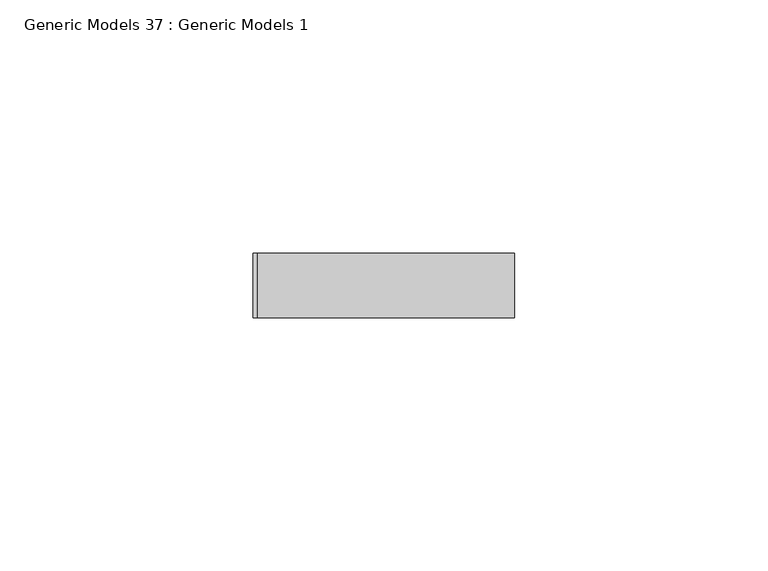
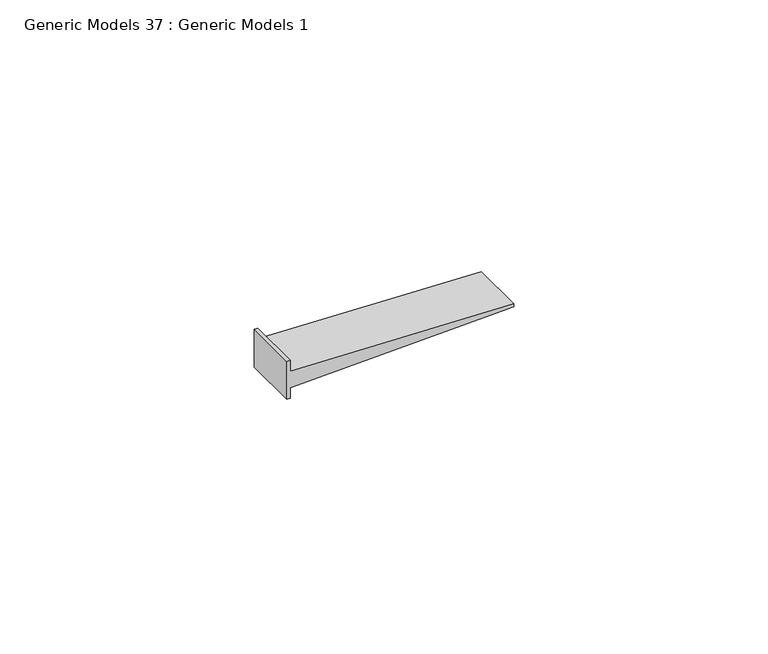
"""IFC4 building model written with IfcOpenShell, lengths in millimetres: proxy geometry, Generic Models 37 : Generic Models 1."""

import ifcopenshell
import ifcopenshell.guid

model = None  # the IFC model being written
_history = None  # IfcOwnerHistory: only IFC2X3 demands one
_inside = {}  # id of a spatial element -> (the spatial element, [elements in it])
_under = {}  # id of a project, library or spatial element -> (it, [spatial elements below it])
_declared = {}  # id of a project -> (the project, [libraries it declares])
_typed = {}  # id of a type object -> (the type object, [elements of that type])
_made_of = {}  # id of a material, layer set ... -> (it, [elements and type objects made of it])


def new_model(schema):
    """Start an empty IFC model of exactly this schema.

    Asked for "IFC4X3", IfcOpenShell would pick the latest addendum, in which some entities
    have other attributes; the version numbers below select the first issue.
    IFC2X3 requires an IfcOwnerHistory on every rooted entity: one is made here for all.
    """
    global model, _history
    if schema == "IFC4X3":
        model = ifcopenshell.file(schema_version=(4, 3, 0, 0))
    else:
        model = ifcopenshell.file(schema=schema)
    _inside.clear()
    _under.clear()
    _declared.clear()
    _typed.clear()
    _made_of.clear()
    _history = None
    if model.schema == "IFC2X3":
        org = make("IfcOrganization", Name="unknown")
        user = make(
            "IfcPersonAndOrganization",
            ThePerson=make("IfcPerson", FamilyName="unknown"),
            TheOrganization=org,
        )
        app = make(
            "IfcApplication",
            ApplicationDeveloper=org,
            Version="unknown",
            ApplicationFullName="unknown",
            ApplicationIdentifier="unknown",
        )
        _history = make(
            "IfcOwnerHistory",
            OwningUser=user,
            OwningApplication=app,
            ChangeAction="ADDED",
            CreationDate=0,
        )
    return model


def make(cls, **values):
    """One entity of the class cls with the attributes given. An attribute that is None is left unset."""
    return model.create_entity(
        cls, **{name: value for name, value in values.items() if value is not None}
    )


def rooted(cls, **values):
    """An entity with a GlobalId (a new one), such as an element, a storey or a relation."""
    return make(cls, GlobalId=ifcopenshell.guid.new(), OwnerHistory=_history, **values)


def si_unit(unit_type, name, prefix=None):
    """IfcSIUnit, for example si_unit("LENGTHUNIT", "METRE", prefix="MILLI")."""
    return make("IfcSIUnit", UnitType=unit_type, Prefix=prefix, Name=name)


def assignment(units):
    """IfcUnitAssignment: the units of a project."""
    return None if units is None else make("IfcUnitAssignment", Units=units)


def point(xyz):
    """IfcCartesianPoint."""
    return None if xyz is None else make("IfcCartesianPoint", Coordinates=xyz)


def direction(xyz):
    """IfcDirection."""
    return None if xyz is None else make("IfcDirection", DirectionRatios=xyz)


def frame(location, z_axis=None, x_axis=None):
    """IfcAxis2Placement3D, a coordinate frame: its origin and axes. An axis left out is left unset."""
    return make(
        "IfcAxis2Placement3D",
        Location=point(location),
        Axis=direction(z_axis),
        RefDirection=direction(x_axis),
    )


def origin():
    """The frame at (0, 0, 0) with its axes left unset."""
    return frame((0.0, 0.0, 0.0))


def place(relative_to, where):
    """IfcLocalPlacement: puts the frame where relative to a parent placement (None: the world)."""
    return make(
        "IfcLocalPlacement", PlacementRelTo=relative_to, RelativePlacement=where
    )


def context(
    kind, dimensions, precision=None, world=None, true_north=None, identifier=None
):
    """IfcGeometricRepresentationContext, for example the 3D "Model" context."""
    return make(
        "IfcGeometricRepresentationContext",
        ContextIdentifier=identifier,
        ContextType=kind,
        CoordinateSpaceDimension=dimensions,
        Precision=precision,
        WorldCoordinateSystem=world,
        TrueNorth=true_north,
    )


def project(units=None, contexts=None):
    """IfcProject with its units and contexts."""
    return rooted(
        "IfcProject",
        Name="project",
        RepresentationContexts=contexts,
        UnitsInContext=assignment(units),
    )


def spatial(cls, under=None, at=None, **own):
    """A site, building, storey or space (cls), placed at a placement, below another one or the project."""
    s = rooted(cls, ObjectPlacement=at, **own)
    if under is not None:
        _under.setdefault(under.id(), (under, []))[1].append(s)
    return s


def polyline(points):
    """IfcPolyline through the points."""
    return make("IfcPolyline", Points=[point(p) for p in points])


def outline(outer, holes=None, kind="AREA"):
    """IfcArbitraryClosedProfileDef: a profile drawn as a closed curve; with holes, ...WithVoids."""
    if holes is None:
        return make("IfcArbitraryClosedProfileDef", ProfileType=kind, OuterCurve=outer)
    return make(
        "IfcArbitraryProfileDefWithVoids",
        ProfileType=kind,
        OuterCurve=outer,
        InnerCurves=holes,
    )


def extrude(swept, where, along, depth):
    """IfcExtrudedAreaSolid: the profile swept, set in the frame where, extruded along a direction by depth."""
    return make(
        "IfcExtrudedAreaSolid",
        SweptArea=swept,
        Position=where,
        ExtrudedDirection=direction(along),
        Depth=depth,
    )


def shape(context_of_items, identifier, shape_type, items):
    """IfcShapeRepresentation: the items that make up one representation, for example the "Body"."""
    return make(
        "IfcShapeRepresentation",
        ContextOfItems=context_of_items,
        RepresentationIdentifier=identifier,
        RepresentationType=shape_type,
        Items=items,
    )


def source(mapping_origin, context_of_items, identifier, shape_type, items):
    """IfcRepresentationMap: a shape defined once, which mapped items show again and again."""
    return make(
        "IfcRepresentationMap",
        MappingOrigin=mapping_origin,
        MappedRepresentation=shape(context_of_items, identifier, shape_type, items),
    )


def transform(
    local_origin,
    x_axis=None,
    y_axis=None,
    z_axis=None,
    scale=None,
    scale2=None,
    scale3=None,
    uniform=True,
):
    """IfcCartesianTransformationOperator3D, or its non-uniform kind. x_axis, y_axis, z_axis: its Axis1, 2, 3."""
    if uniform:
        return make(
            "IfcCartesianTransformationOperator3D",
            Axis1=direction(x_axis),
            Axis2=direction(y_axis),
            LocalOrigin=point(local_origin),
            Scale=scale,
            Axis3=direction(z_axis),
        )
    return make(
        "IfcCartesianTransformationOperator3DnonUniform",
        Axis1=direction(x_axis),
        Axis2=direction(y_axis),
        LocalOrigin=point(local_origin),
        Scale=scale,
        Axis3=direction(z_axis),
        Scale2=scale2,
        Scale3=scale3,
    )


def mapped(mapping_source, mapping_target):
    """IfcMappedItem: shows the shape of a source again, moved by a transform."""
    return make(
        "IfcMappedItem", MappingSource=mapping_source, MappingTarget=mapping_target
    )


def made_of(thing, what):
    """Note that an element or type object is made of a material, layer set ...; save() writes the relation."""
    if what is not None:
        _made_of.setdefault(what.id(), (what, []))[1].append(thing)
    return thing


def element(
    cls,
    number,
    at=None,
    inside=None,
    cuts=None,
    type_object=None,
    material=None,
    context=None,
    identifier="Body",
    shape_type=None,
    held_by="IfcProductDefinitionShape",
    body=None,
    shapes=None,
    **own,
):
    """One element of the class cls, such as IfcWall. Its Tag is "e" and its number.

    at: its placement. inside: the storey or other place that contains it. cuts: it is an
    opening in that element (IfcRelVoidsElement). A single representation is given by context,
    identifier, shape_type and body (its items); several are given by shapes. held_by: the class
    of the entity that holds the representations. save() writes the other relations.
    """
    e = rooted(cls, Tag="e%d" % number, ObjectPlacement=at, **own)
    if body is not None:
        shapes = [shape(context, identifier, shape_type, body)]
    if shapes is not None:
        e.Representation = make(held_by, Representations=shapes)
    if inside is not None:
        _inside.setdefault(inside.id(), (inside, []))[1].append(e)
    if cuts is not None:
        rooted(
            "IfcRelVoidsElement", RelatingBuildingElement=cuts, RelatedOpeningElement=e
        )
    if type_object is not None:
        _typed.setdefault(type_object.id(), (type_object, []))[1].append(e)
    return made_of(e, material)


def aggregate(whole, parts):
    """IfcRelAggregates: a whole, such as a stair, and the parts it consists of."""
    return rooted("IfcRelAggregates", RelatingObject=whole, RelatedObjects=parts)


def save(model, path):
    """Write the relations noted so far, then the file.

    IfcRelAggregates (storeys below a building ...), IfcRelContainedInSpatialStructure (elements
    in a storey), IfcRelDefinesByType, IfcRelAssociatesMaterial and IfcRelDeclares: one each for
    every whole, place, type object, material and project.
    """
    for whole, parts in _under.values():
        aggregate(whole, parts)
    for where, things in _inside.values():
        rooted(
            "IfcRelContainedInSpatialStructure",
            RelatedElements=things,
            RelatingStructure=where,
        )
    for kind, things in _typed.values():
        rooted("IfcRelDefinesByType", RelatedObjects=things, RelatingType=kind)
    for what, things in _made_of.values():
        rooted("IfcRelAssociatesMaterial", RelatedObjects=things, RelatingMaterial=what)
    for by, libraries in _declared.values():
        rooted("IfcRelDeclares", RelatingContext=by, RelatedDefinitions=libraries)
    model.write(path)


def generic_models_37_generic_models_1_916dd7c6(model_context):
    return source(origin(), model_context, "Body", "SweptSolid", [
        extrude(outline(polyline([(2409.6091, 49675.25625), (2400.5159, 49675.25625), (2400.5159, 49676.05), (2403.0657636, 49676.05), (2404.6631527, 49726.85), (2405.4618473, 49726.85), (2407.0592364, 49676.05), (2409.6091, 49676.05), (2409.6091, 49675.25625)])), frame((0.0, 565.15, 0.0), z_axis=(0.0, 1.0, 0.0), x_axis=(0.0, 0.0, 1.0)), (0.0, 0.0, 1.0), 12.7),
    ])


if __name__ == "__main__":
    model = new_model("IFC4")
    model_context = context("Model", 3, world=origin())
    ifc_project = project(units=[si_unit("LENGTHUNIT", "METRE", prefix="MILLI")], contexts=[model_context])
    site = spatial("IfcSite", under=ifc_project)
    building = spatial("IfcBuilding", under=site)
    placement = place(None, origin())
    generic_models_37_generic_models_1_shape = generic_models_37_generic_models_1_916dd7c6(model_context)
    element("IfcBuildingElementProxy", 1, Name="Generic Models 37 : Generic Models 1", ObjectType="Generic Models 37 : Generic Models 1", at=placement, inside=building, context=model_context, shape_type="MappedRepresentation", body=[
        mapped(generic_models_37_generic_models_1_shape, transform((0.0, 0.0, 0.0), x_axis=(1.0, 0.0, 0.0), y_axis=(0.0, 1.0, 0.0), z_axis=(0.0, 0.0, 1.0))),
    ])
    save(model, "model.ifc")

# Revit data of these elements
# Element 1 (IfcBuildingElementProxy, "Generic Models 37 : Generic Models 1")
#   Materials on its faces: "ATTACH GYPSUM BOARD TO STUDS AND NOT TO TOP TRACK"
# Materials
#   "ATTACH GYPSUM BOARD TO STUDS AND NOT TO TOP TRACK": class "Generic", colour RGB 48 48 48, transparency 0, Cost = 0
